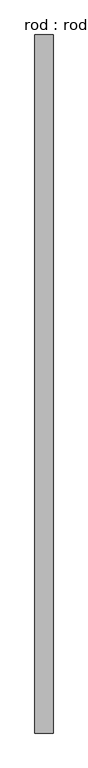
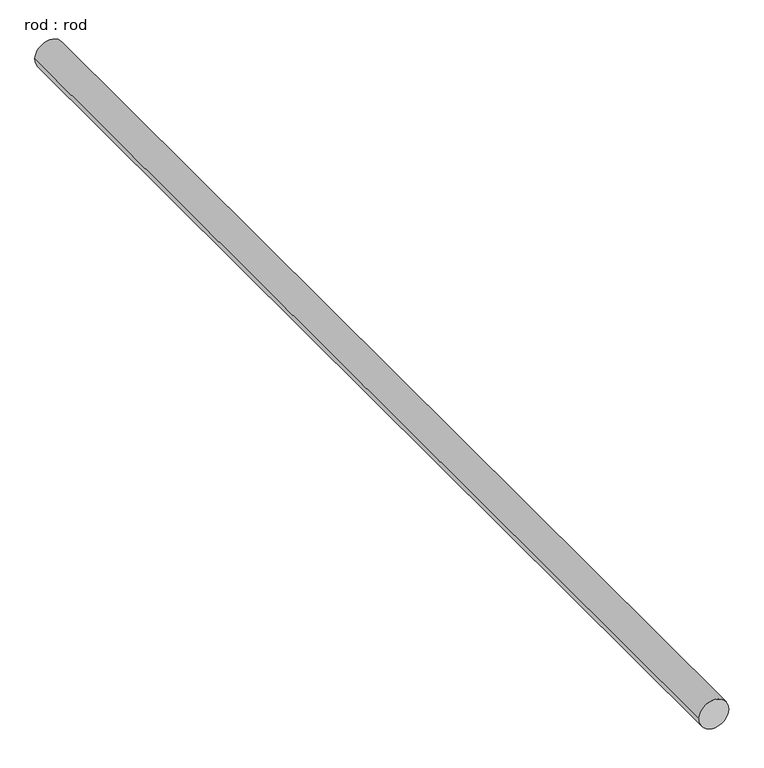
"""IFC4 building model written with IfcOpenShell, lengths in millimetres: proxy geometry, rod : rod."""

from ifc_helpers import new_model, si_unit, point, frame, frame_2d, origin, place, context, project, spatial, circle_curve, trimmed, segment, composite_curve, outline, extrude, source, transform, mapped, element, save


def rod_rod_8dcea08d(model_context):
    return source(origin(), model_context, "Body", "SweptSolid", [
        extrude(outline(composite_curve([segment(trimmed(circle_curve(frame_2d((0.0108462, 0.0)), 200.0), [point((0.0108462, 200.0))], [point((0.0108462, -200.0))], False, "CARTESIAN"), True, "CONTINUOUS"), segment(trimmed(circle_curve(frame_2d((0.0108462, 0.0)), 200.0), [point((0.0108462, -200.0))], [point((0.0108462, 200.0))], False, "CARTESIAN"), True, "CONTINUOUS")], self_intersect=False)), frame((0.0, -3594.7713847, 0.0), z_axis=(0.0, 1.0, 0.0), x_axis=(0.0, 0.0, 1.0)), (0.0, 0.0, 1.0), 15375.0),
    ])


if __name__ == "__main__":
    model = new_model("IFC4")
    model_context = context("Model", 3, world=origin())
    ifc_project = project(units=[si_unit("LENGTHUNIT", "METRE", prefix="MILLI")], contexts=[model_context])
    site = spatial("IfcSite", under=ifc_project)
    building = spatial("IfcBuilding", under=site)
    placement = place(None, origin())
    rod_rod_shape = rod_rod_8dcea08d(model_context)
    element("IfcBuildingElementProxy", 1, Name="rod : rod", ObjectType="rod : rod", at=placement, inside=building, context=model_context, shape_type="MappedRepresentation", body=[
        mapped(rod_rod_shape, transform((0.0, 0.0, 0.0), x_axis=(1.0, 0.0, 0.0), y_axis=(0.0, 1.0, 0.0), z_axis=(0.0, 0.0, 1.0))),
    ])
    save(model, "model.ifc")

# Revit data of these elements
# Type "rod : rod"
#   Default Elevation = 0
